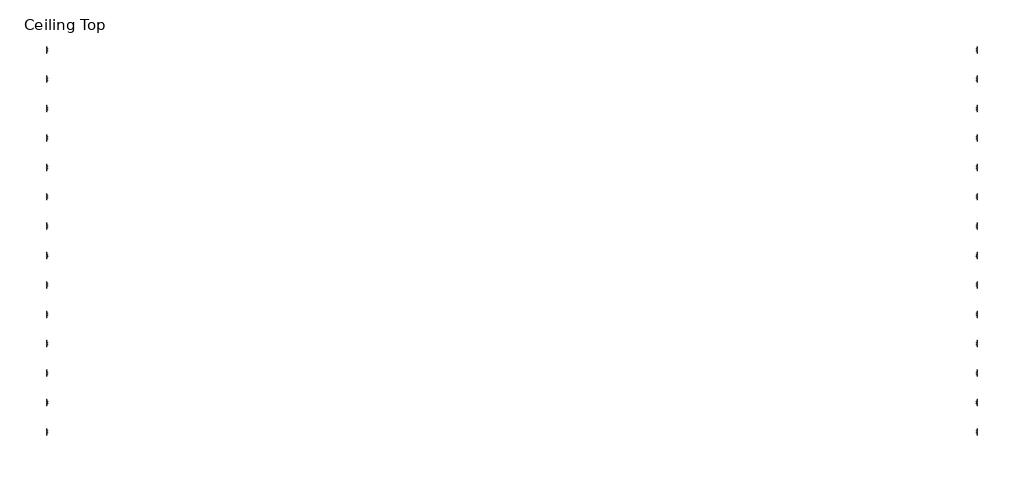
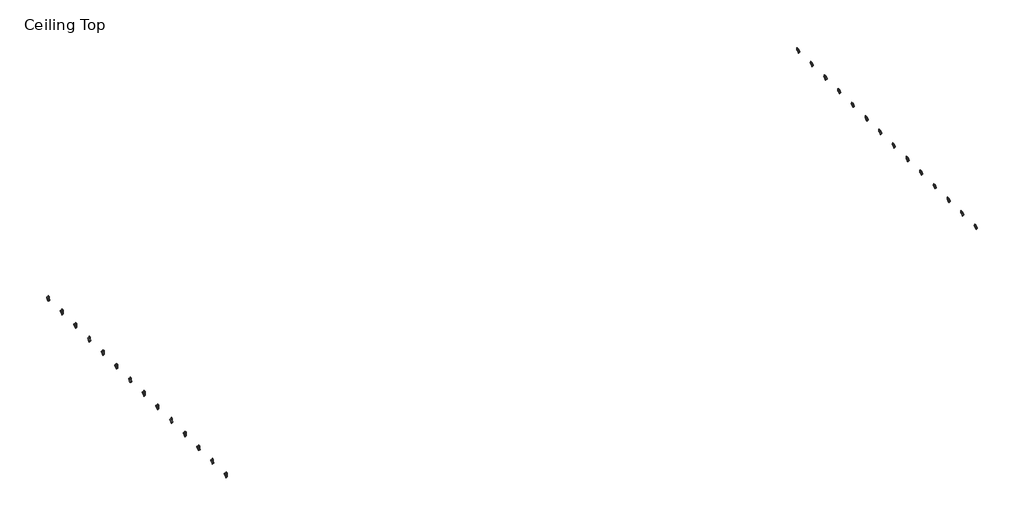
# One storey: 28 proxies.
"""IFC4 building model written with IfcOpenShell, lengths in millimetres."""

import ifcopenshell
import ifcopenshell.guid

model = None  # the IFC model being written
_history = None  # IfcOwnerHistory: only IFC2X3 demands one
_inside = {}  # id of a spatial element -> (the spatial element, [elements in it])
_under = {}  # id of a project, library or spatial element -> (it, [spatial elements below it])
_declared = {}  # id of a project -> (the project, [libraries it declares])
_typed = {}  # id of a type object -> (the type object, [elements of that type])
_made_of = {}  # id of a material, layer set ... -> (it, [elements and type objects made of it])


def new_model(schema):
    """Start an empty IFC model of exactly this schema.

    Asked for "IFC4X3", IfcOpenShell would pick the latest addendum, in which some entities
    have other attributes; the version numbers below select the first issue.
    IFC2X3 requires an IfcOwnerHistory on every rooted entity: one is made here for all.
    """
    global model, _history
    if schema == "IFC4X3":
        model = ifcopenshell.file(schema_version=(4, 3, 0, 0))
    else:
        model = ifcopenshell.file(schema=schema)
    _inside.clear()
    _under.clear()
    _declared.clear()
    _typed.clear()
    _made_of.clear()
    _history = None
    if model.schema == "IFC2X3":
        org = make("IfcOrganization", Name="unknown")
        user = make(
            "IfcPersonAndOrganization",
            ThePerson=make("IfcPerson", FamilyName="unknown"),
            TheOrganization=org,
        )
        app = make(
            "IfcApplication",
            ApplicationDeveloper=org,
            Version="unknown",
            ApplicationFullName="unknown",
            ApplicationIdentifier="unknown",
        )
        _history = make(
            "IfcOwnerHistory",
            OwningUser=user,
            OwningApplication=app,
            ChangeAction="ADDED",
            CreationDate=0,
        )
    return model


def make(cls, **values):
    """One entity of the class cls with the attributes given. An attribute that is None is left unset."""
    return model.create_entity(
        cls, **{name: value for name, value in values.items() if value is not None}
    )


def rooted(cls, **values):
    """An entity with a GlobalId (a new one), such as an element, a storey or a relation."""
    return make(cls, GlobalId=ifcopenshell.guid.new(), OwnerHistory=_history, **values)


def si_unit(unit_type, name, prefix=None):
    """IfcSIUnit, for example si_unit("LENGTHUNIT", "METRE", prefix="MILLI")."""
    return make("IfcSIUnit", UnitType=unit_type, Prefix=prefix, Name=name)


def assignment(units):
    """IfcUnitAssignment: the units of a project."""
    return None if units is None else make("IfcUnitAssignment", Units=units)


def point(xyz):
    """IfcCartesianPoint."""
    return None if xyz is None else make("IfcCartesianPoint", Coordinates=xyz)


def direction(xyz):
    """IfcDirection."""
    return None if xyz is None else make("IfcDirection", DirectionRatios=xyz)


def frame(location, z_axis=None, x_axis=None):
    """IfcAxis2Placement3D, a coordinate frame: its origin and axes. An axis left out is left unset."""
    return make(
        "IfcAxis2Placement3D",
        Location=point(location),
        Axis=direction(z_axis),
        RefDirection=direction(x_axis),
    )


def origin():
    """The frame at (0, 0, 0) with its axes left unset."""
    return frame((0.0, 0.0, 0.0))


def place(relative_to, where):
    """IfcLocalPlacement: puts the frame where relative to a parent placement (None: the world)."""
    return make(
        "IfcLocalPlacement", PlacementRelTo=relative_to, RelativePlacement=where
    )


def context(
    kind, dimensions, precision=None, world=None, true_north=None, identifier=None
):
    """IfcGeometricRepresentationContext, for example the 3D "Model" context."""
    return make(
        "IfcGeometricRepresentationContext",
        ContextIdentifier=identifier,
        ContextType=kind,
        CoordinateSpaceDimension=dimensions,
        Precision=precision,
        WorldCoordinateSystem=world,
        TrueNorth=true_north,
    )


def project(units=None, contexts=None):
    """IfcProject with its units and contexts."""
    return rooted(
        "IfcProject",
        Name="project",
        RepresentationContexts=contexts,
        UnitsInContext=assignment(units),
    )


def spatial(cls, under=None, at=None, **own):
    """A site, building, storey or space (cls), placed at a placement, below another one or the project."""
    s = rooted(cls, ObjectPlacement=at, **own)
    if under is not None:
        _under.setdefault(under.id(), (under, []))[1].append(s)
    return s


def polyline(points):
    """IfcPolyline through the points."""
    return make("IfcPolyline", Points=[point(p) for p in points])


def circle_curve(where, radius):
    """IfcCircle in the frame where."""
    return make("IfcCircle", Position=where, Radius=radius)


def shape(context_of_items, identifier, shape_type, items):
    """IfcShapeRepresentation: the items that make up one representation, for example the "Body"."""
    return make(
        "IfcShapeRepresentation",
        ContextOfItems=context_of_items,
        RepresentationIdentifier=identifier,
        RepresentationType=shape_type,
        Items=items,
    )


def source(mapping_origin, context_of_items, identifier, shape_type, items):
    """IfcRepresentationMap: a shape defined once, which mapped items show again and again."""
    return make(
        "IfcRepresentationMap",
        MappingOrigin=mapping_origin,
        MappedRepresentation=shape(context_of_items, identifier, shape_type, items),
    )


def transform(
    local_origin,
    x_axis=None,
    y_axis=None,
    z_axis=None,
    scale=None,
    scale2=None,
    scale3=None,
    uniform=True,
):
    """IfcCartesianTransformationOperator3D, or its non-uniform kind. x_axis, y_axis, z_axis: its Axis1, 2, 3."""
    if uniform:
        return make(
            "IfcCartesianTransformationOperator3D",
            Axis1=direction(x_axis),
            Axis2=direction(y_axis),
            LocalOrigin=point(local_origin),
            Scale=scale,
            Axis3=direction(z_axis),
        )
    return make(
        "IfcCartesianTransformationOperator3DnonUniform",
        Axis1=direction(x_axis),
        Axis2=direction(y_axis),
        LocalOrigin=point(local_origin),
        Scale=scale,
        Axis3=direction(z_axis),
        Scale2=scale2,
        Scale3=scale3,
    )


def mapped(mapping_source, mapping_target):
    """IfcMappedItem: shows the shape of a source again, moved by a transform."""
    return make(
        "IfcMappedItem", MappingSource=mapping_source, MappingTarget=mapping_target
    )


def made_of(thing, what):
    """Note that an element or type object is made of a material, layer set ...; save() writes the relation."""
    if what is not None:
        _made_of.setdefault(what.id(), (what, []))[1].append(thing)
    return thing


def element(
    cls,
    number,
    at=None,
    inside=None,
    cuts=None,
    type_object=None,
    material=None,
    context=None,
    identifier="Body",
    shape_type=None,
    held_by="IfcProductDefinitionShape",
    body=None,
    shapes=None,
    **own,
):
    """One element of the class cls, such as IfcWall. Its Tag is "e" and its number.

    at: its placement. inside: the storey or other place that contains it. cuts: it is an
    opening in that element (IfcRelVoidsElement). A single representation is given by context,
    identifier, shape_type and body (its items); several are given by shapes. held_by: the class
    of the entity that holds the representations. save() writes the other relations.
    """
    e = rooted(cls, Tag="e%d" % number, ObjectPlacement=at, **own)
    if body is not None:
        shapes = [shape(context, identifier, shape_type, body)]
    if shapes is not None:
        e.Representation = make(held_by, Representations=shapes)
    if inside is not None:
        _inside.setdefault(inside.id(), (inside, []))[1].append(e)
    if cuts is not None:
        rooted(
            "IfcRelVoidsElement", RelatingBuildingElement=cuts, RelatedOpeningElement=e
        )
    if type_object is not None:
        _typed.setdefault(type_object.id(), (type_object, []))[1].append(e)
    return made_of(e, material)


def aggregate(whole, parts):
    """IfcRelAggregates: a whole, such as a stair, and the parts it consists of."""
    return rooted("IfcRelAggregates", RelatingObject=whole, RelatedObjects=parts)


def save(model, path):
    """Write the relations noted so far, then the file.

    IfcRelAggregates (storeys below a building ...), IfcRelContainedInSpatialStructure (elements
    in a storey), IfcRelDefinesByType, IfcRelAssociatesMaterial and IfcRelDeclares: one each for
    every whole, place, type object, material and project.
    """
    for whole, parts in _under.values():
        aggregate(whole, parts)
    for where, things in _inside.values():
        rooted(
            "IfcRelContainedInSpatialStructure",
            RelatedElements=things,
            RelatingStructure=where,
        )
    for kind, things in _typed.values():
        rooted("IfcRelDefinesByType", RelatedObjects=things, RelatingType=kind)
    for what, things in _made_of.values():
        rooted("IfcRelAssociatesMaterial", RelatedObjects=things, RelatingMaterial=what)
    for by, libraries in _declared.values():
        rooted("IfcRelDeclares", RelatingContext=by, RelatedDefinitions=libraries)
    model.write(path)


def plane_surface(at):
    """IfcPlane: the flat surface through the origin of the frame at, square to its z axis."""
    return make("IfcPlane", Position=at)


def revolved_surface(curve, axis_point, axis_direction):
    """IfcSurfaceOfRevolution: the curve turned about the line through axis_point along axis_direction."""
    return make(
        "IfcSurfaceOfRevolution",
        SweptCurve=make("IfcArbitraryOpenProfileDef", ProfileType="CURVE", Curve=curve),
        AxisPosition=make("IfcAxis1Placement", Location=point(axis_point), Axis=direction(axis_direction)),
    )


def advanced_brep(points, edges, surfaces, faces):
    """IfcAdvancedBrep: a solid bounded by faces that lie on surfaces and meet in shared edges.

    An edge is (start, end): straight between two places in points (the first is 0);
    or (start, end, curve); or (start, end, curve, False) where it runs against its curve.
    A face is (place in surfaces, loops), or (place, loops, False) where it looks against
    its surface's normal. A loop lists edges by number (the first is 1), with a minus sign
    where the edge is run from its end to its start. The first loop is the outer one.
    """
    corners = [point(p) for p in points]
    vertices = [make("IfcVertexPoint", VertexGeometry=c) for c in corners]
    made = []
    for start, end, *more in edges:
        made.append(
            make(
                "IfcEdgeCurve",
                EdgeStart=vertices[start],
                EdgeEnd=vertices[end],
                EdgeGeometry=more[0] if more else make("IfcPolyline", Points=[corners[start], corners[end]]),
                SameSense=more[1] if len(more) > 1 else True,
            )
        )
    hull = []
    for where, loops, *sense in faces:
        bounds = []
        for j, loop in enumerate(loops):
            ring = [make("IfcOrientedEdge", EdgeElement=made[abs(k) - 1], Orientation=k > 0) for k in loop]
            bounds.append(
                make(
                    "IfcFaceOuterBound" if j == 0 else "IfcFaceBound",
                    Bound=make("IfcEdgeLoop", EdgeList=ring),
                    Orientation=True,
                )
            )
        hull.append(make("IfcAdvancedFace", Bounds=bounds, FaceSurface=surfaces[where], SameSense=sense[0] if sense else True))
    return make("IfcAdvancedBrep", Outer=make("IfcClosedShell", CfsFaces=hull))


def generic_models_343c88cb(model_context):
    return source(origin(), model_context, "Body", "AdvancedBrep", [
        advanced_brep(
        [(-0.790575, 0.0, 54.76875), (3.171825, 0.0, 54.76875), (3.171825, 1.18872, 54.76875), (-0.790575, 1.18872, 54.76875), (-0.790575, 0.0, 16.66875), (3.171825, 0.0, 16.66875), (3.171825, 1.18872, 16.66875), (-0.790575, 1.18872, 16.66875), (43.659425, 0.0, 10.31875), (47.621825, 0.0, 10.31875), (47.621825, 1.18872, 10.31875), (43.659425, 1.18872, 10.31875), (-45.240575, 0.0, 10.31875), (-41.278175, 0.0, 10.31875), (-41.278175, 1.18872, 10.31875), (-45.240575, 1.18872, 10.31875), (19.84756, 11.902103, -19.05), (19.84756, 15.864503, -19.05), (21.03628, 15.864503, -19.05), (21.03628, 11.902103, -19.05), (19.84756, 11.902103, -36.5125), (19.84756, 15.864503, -36.5125), (21.03628, 15.864503, -36.5125), (21.03628, 11.902103, -36.5125), (19.84756, 11.902103, -53.975), (19.84756, 15.864503, -53.975), (21.03628, 15.864503, -53.975), (21.03628, 11.902103, -53.975), (-21.03628, 11.902103, -57.15), (-21.03628, 15.864503, -57.15), (-19.84756, 15.864503, -57.15), (-19.84756, 11.902103, -57.15), (-21.03628, 11.902103, -39.6875), (-21.03628, 15.864503, -39.6875), (-19.84756, 15.864503, -39.6875), (-19.84756, 11.902103, -39.6875), (-21.03628, 11.902103, -22.225), (-21.03628, 15.864503, -22.225), (-19.84756, 15.864503, -22.225), (-19.84756, 11.902103, -22.225), (23.08225, 0.0, 0.0), (23.08225, 1.18872, 0.0), (23.08225, 1.18872, -3.175), (23.08225, 0.0, -3.175), (21.03628, 0.0, -56.758894), (19.84756, 0.0, -56.758894), (19.84756, 1.698923, -56.758894), (21.03628, 1.698923, -56.758894), (21.03628, 1.18872, -56.758894), (19.84756, 0.0, -3.175), (21.03628, 1.18872, -3.175), (21.03628, 21.820803, -3.175), (19.84756, 21.820803, -3.175), (-23.08225, 1.18872, 0.0), (-23.08225, 1.18872, -3.175), (-21.03628, 1.18872, -3.175), (-21.03628, 1.18872, -56.758894), (-67.071875, 1.18872, -10.723299), (-67.071875, 1.18872, -1.182951), (-4.770174, 1.18872, 61.11875), (4.770174, 1.18872, 61.11875), (67.071875, 1.18872, -1.182951), (67.071875, 1.18872, -10.723299), (19.84756, 21.820803, -73.025), (19.84756, 17.965029, -73.025), (-21.03628, 1.698923, -56.758894), (-19.84756, 1.698923, -56.758894), (-19.84756, 0.0, -56.758894), (-21.03628, 0.0, -56.758894), (67.071875, 0.0, -10.723299), (67.071875, 0.0, -1.182951), (4.770174, 0.0, 61.11875), (-4.770174, 0.0, 61.11875), (-67.071875, 0.0, -1.182951), (-67.071875, 0.0, -10.723299), (-19.84756, 0.0, -3.175), (-23.08225, 0.0, -3.175), (-23.08225, 0.0, 0.0), (-19.84756, 21.820803, -3.175), (-21.03628, 21.820803, -3.175), (21.03628, 17.965029, -73.025), (21.03628, 21.820803, -73.025), (-19.84756, 17.965029, -73.025), (-19.84756, 21.820803, -73.025), (-21.03628, 21.820803, -73.025), (-21.03628, 17.965029, -73.025)],
        [
            (0, 1, circle_curve(frame((1.190625, 0.0, 54.76875), z_axis=(0.0, -1.0, 0.0), x_axis=(-1.0, 0.0, 0.0)), 1.9812)),
            (1, 2),
            (2, 3, circle_curve(frame((1.190625, 1.18872, 54.76875), z_axis=(0.0, 1.0, 0.0), x_axis=(-1.0, 0.0, 0.0)), 1.9812)),
            (3, 0),
            (4, 5, circle_curve(frame((1.190625, 0.0, 16.66875), z_axis=(0.0, -1.0, 0.0), x_axis=(-1.0, 0.0, 0.0)), 1.9812)),
            (5, 6),
            (6, 7, circle_curve(frame((1.190625, 1.18872, 16.66875), z_axis=(0.0, 1.0, 0.0), x_axis=(-1.0, 0.0, 0.0)), 1.9812)),
            (7, 4),
            (8, 9, circle_curve(frame((45.640625, 0.0, 10.31875), z_axis=(0.0, -1.0, 0.0), x_axis=(-1.0, 0.0, 0.0)), 1.9812)),
            (9, 10),
            (10, 11, circle_curve(frame((45.640625, 1.18872, 10.31875), z_axis=(0.0, 1.0, 0.0), x_axis=(-1.0, 0.0, 0.0)), 1.9812)),
            (11, 8),
            (12, 13, circle_curve(frame((-43.259375, 0.0, 10.31875), z_axis=(0.0, -1.0, 0.0), x_axis=(-1.0, 0.0, 0.0)), 1.9812)),
            (13, 14),
            (14, 15, circle_curve(frame((-43.259375, 1.18872, 10.31875), z_axis=(0.0, 1.0, 0.0), x_axis=(-1.0, 0.0, 0.0)), 1.9812)),
            (15, 12),
            (16, 17, circle_curve(frame((19.84756, 13.883303, -19.05), z_axis=(-1.0, 0.0, 0.0), x_axis=(0.0, -1.0, 0.0)), 1.9812)),
            (17, 18),
            (18, 19, circle_curve(frame((21.03628, 13.883303, -19.05), z_axis=(1.0, 0.0, 0.0), x_axis=(0.0, -1.0, 0.0)), 1.9812)),
            (19, 16),
            (20, 21, circle_curve(frame((19.84756, 13.883303, -36.5125), z_axis=(-1.0, 0.0, 0.0), x_axis=(0.0, -1.0, 0.0)), 1.9812)),
            (21, 22),
            (22, 23, circle_curve(frame((21.03628, 13.883303, -36.5125), z_axis=(1.0, 0.0, 0.0), x_axis=(0.0, -1.0, 0.0)), 1.9812)),
            (23, 20),
            (24, 25, circle_curve(frame((19.84756, 13.883303, -53.975), z_axis=(-1.0, 0.0, 0.0), x_axis=(0.0, -1.0, 0.0)), 1.9812)),
            (25, 26),
            (26, 27, circle_curve(frame((21.03628, 13.883303, -53.975), z_axis=(1.0, 0.0, 0.0), x_axis=(0.0, -1.0, 0.0)), 1.9812)),
            (27, 24),
            (28, 29, circle_curve(frame((-21.03628, 13.883303, -57.15), z_axis=(-1.0, 0.0, 0.0), x_axis=(0.0, -1.0, 0.0)), 1.9812)),
            (29, 30),
            (30, 31, circle_curve(frame((-19.84756, 13.883303, -57.15), z_axis=(1.0, 0.0, 0.0), x_axis=(0.0, -1.0, 0.0)), 1.9812)),
            (31, 28),
            (32, 33, circle_curve(frame((-21.03628, 13.883303, -39.6875), z_axis=(-1.0, 0.0, 0.0), x_axis=(0.0, -1.0, 0.0)), 1.9812)),
            (33, 34),
            (34, 35, circle_curve(frame((-19.84756, 13.883303, -39.6875), z_axis=(1.0, 0.0, 0.0), x_axis=(0.0, -1.0, 0.0)), 1.9812)),
            (35, 32),
            (36, 37, circle_curve(frame((-21.03628, 13.883303, -22.225), z_axis=(-1.0, 0.0, 0.0), x_axis=(0.0, -1.0, 0.0)), 1.9812)),
            (37, 38),
            (38, 39, circle_curve(frame((-19.84756, 13.883303, -22.225), z_axis=(1.0, 0.0, 0.0), x_axis=(0.0, -1.0, 0.0)), 1.9812)),
            (39, 36),
            (40, 41),
            (41, 42),
            (42, 43),
            (43, 40),
            (44, 45),
            (45, 46),
            (46, 47),
            (47, 48),
            (48, 44),
            (49, 43),
            (42, 50),
            (50, 51),
            (51, 52),
            (52, 49),
            (53, 54),
            (54, 55),
            (55, 56),
            (56, 57),
            (57, 58),
            (58, 59),
            (59, 60),
            (60, 61),
            (61, 62),
            (62, 48),
            (48, 50),
            (41, 53),
            (14, 15, circle_curve(frame((-43.259375, 1.18872, 10.31875), z_axis=(0.0, -1.0, 0.0), x_axis=(-1.0, 0.0, 0.0)), 1.9812)),
            (10, 11, circle_curve(frame((45.640625, 1.18872, 10.31875), z_axis=(0.0, -1.0, 0.0), x_axis=(-1.0, 0.0, 0.0)), 1.9812)),
            (6, 7, circle_curve(frame((1.190625, 1.18872, 16.66875), z_axis=(0.0, -1.0, 0.0), x_axis=(-1.0, 0.0, 0.0)), 1.9812)),
            (2, 3, circle_curve(frame((1.190625, 1.18872, 54.76875), z_axis=(0.0, -1.0, 0.0), x_axis=(-1.0, 0.0, 0.0)), 1.9812)),
            (45, 49),
            (52, 63),
            (63, 64),
            (64, 46),
            (16, 17, circle_curve(frame((19.84756, 13.883303, -19.05), z_axis=(1.0, 0.0, 0.0), x_axis=(0.0, -1.0, 0.0)), 1.9812)),
            (20, 21, circle_curve(frame((19.84756, 13.883303, -36.5125), z_axis=(1.0, 0.0, 0.0), x_axis=(0.0, -1.0, 0.0)), 1.9812)),
            (24, 25, circle_curve(frame((19.84756, 13.883303, -53.975), z_axis=(1.0, 0.0, 0.0), x_axis=(0.0, -1.0, 0.0)), 1.9812)),
            (56, 65),
            (65, 66),
            (66, 67),
            (67, 68),
            (68, 56),
            (44, 69),
            (69, 70),
            (70, 71),
            (71, 72),
            (72, 73),
            (73, 74),
            (74, 68),
            (67, 75),
            (75, 76),
            (76, 77),
            (77, 40),
            (0, 1, circle_curve(frame((1.190625, 0.0, 54.76875), z_axis=(0.0, 1.0, 0.0), x_axis=(-1.0, 0.0, 0.0)), 1.9812)),
            (4, 5, circle_curve(frame((1.190625, 0.0, 16.66875), z_axis=(0.0, 1.0, 0.0), x_axis=(-1.0, 0.0, 0.0)), 1.9812)),
            (8, 9, circle_curve(frame((45.640625, 0.0, 10.31875), z_axis=(0.0, 1.0, 0.0), x_axis=(-1.0, 0.0, 0.0)), 1.9812)),
            (12, 13, circle_curve(frame((-43.259375, 0.0, 10.31875), z_axis=(0.0, 1.0, 0.0), x_axis=(-1.0, 0.0, 0.0)), 1.9812)),
            (74, 57),
            (76, 54),
            (53, 77),
            (75, 78),
            (78, 79),
            (79, 55),
            (64, 80),
            (80, 47),
            (80, 81),
            (81, 51),
            (26, 27, circle_curve(frame((21.03628, 13.883303, -53.975), z_axis=(-1.0, 0.0, 0.0), x_axis=(0.0, -1.0, 0.0)), 1.9812)),
            (22, 23, circle_curve(frame((21.03628, 13.883303, -36.5125), z_axis=(-1.0, 0.0, 0.0), x_axis=(0.0, -1.0, 0.0)), 1.9812)),
            (18, 19, circle_curve(frame((21.03628, 13.883303, -19.05), z_axis=(-1.0, 0.0, 0.0), x_axis=(0.0, -1.0, 0.0)), 1.9812)),
            (66, 82),
            (82, 83),
            (83, 78),
            (38, 39, circle_curve(frame((-19.84756, 13.883303, -22.225), z_axis=(-1.0, 0.0, 0.0), x_axis=(0.0, -1.0, 0.0)), 1.9812)),
            (34, 35, circle_curve(frame((-19.84756, 13.883303, -39.6875), z_axis=(-1.0, 0.0, 0.0), x_axis=(0.0, -1.0, 0.0)), 1.9812)),
            (30, 31, circle_curve(frame((-19.84756, 13.883303, -57.15), z_axis=(-1.0, 0.0, 0.0), x_axis=(0.0, -1.0, 0.0)), 1.9812)),
            (79, 84),
            (84, 85),
            (85, 65),
            (28, 29, circle_curve(frame((-21.03628, 13.883303, -57.15), z_axis=(1.0, 0.0, 0.0), x_axis=(0.0, -1.0, 0.0)), 1.9812)),
            (32, 33, circle_curve(frame((-21.03628, 13.883303, -39.6875), z_axis=(1.0, 0.0, 0.0), x_axis=(0.0, -1.0, 0.0)), 1.9812)),
            (36, 37, circle_curve(frame((-21.03628, 13.883303, -22.225), z_axis=(1.0, 0.0, 0.0), x_axis=(0.0, -1.0, 0.0)), 1.9812)),
            (85, 82),
            (72, 59),
            (58, 73),
            (84, 83),
            (81, 63),
            (62, 69),
            (61, 70),
            (60, 71),
        ],
        [
            revolved_surface(polyline([(-0.790575, 0.0, 54.76875), (-0.790575, 1.18872, 54.76875)]), (1.190625, 1.18872, 54.76875), (0.0, -1.0, 0.0)),
            revolved_surface(polyline([(-0.790575, 0.0, 16.66875), (-0.790575, 1.18872, 16.66875)]), (1.190625, 1.18872, 16.66875), (0.0, -1.0, 0.0)),
            revolved_surface(polyline([(43.659425, 0.0, 10.31875), (43.659425, 1.18872, 10.31875)]), (45.640625, 1.18872, 10.31875), (0.0, -1.0, 0.0)),
            revolved_surface(polyline([(-45.240575, 0.0, 10.31875), (-45.240575, 1.18872, 10.31875)]), (-43.259375, 1.18872, 10.31875), (0.0, -1.0, 0.0)),
            revolved_surface(polyline([(19.84756, 11.902103, -19.05), (21.03628, 11.902103, -19.05)]), (21.03628, 13.883303, -19.05), (-1.0, 0.0, 0.0)),
            revolved_surface(polyline([(19.84756, 11.902103, -36.5125), (21.03628, 11.902103, -36.5125)]), (21.03628, 13.883303, -36.5125), (-1.0, 0.0, 0.0)),
            revolved_surface(polyline([(19.84756, 11.902103, -53.975), (21.03628, 11.902103, -53.975)]), (21.03628, 13.883303, -53.975), (-1.0, 0.0, 0.0)),
            revolved_surface(polyline([(-21.03628, 11.902103, -57.15), (-19.84756, 11.902103, -57.15)]), (-19.84756, 13.883303, -57.15), (-1.0, 0.0, 0.0)),
            revolved_surface(polyline([(-21.03628, 11.902103, -39.6875), (-19.84756, 11.902103, -39.6875)]), (-19.84756, 13.883303, -39.6875), (-1.0, 0.0, 0.0)),
            revolved_surface(polyline([(-21.03628, 11.902103, -22.225), (-19.84756, 11.902103, -22.225)]), (-19.84756, 13.883303, -22.225), (-1.0, 0.0, 0.0)),
            plane_surface(frame((23.08225, 1.18872, -3.175), z_axis=(-1.0, 0.0, 0.0), x_axis=(0.0, 0.0, 1.0))),
            plane_surface(frame((19.84756, 0.0, -56.758894), z_axis=(0.0, 0.0, -1.0), x_axis=(1.0, 0.0, 0.0))),
            plane_surface(frame((21.03628, 1.240453, -3.175), z_axis=(0.0, 0.0, 1.0), x_axis=(1.0, 0.0, 0.0))),
            plane_surface(frame((0.0, 1.18872, -12.3047323), z_axis=(0.0, 1.0, 0.0), x_axis=(1.0, 0.0, 0.0))),
            plane_surface(frame((19.84756, 22.735203, -12.3047323), z_axis=(-1.0, 0.0, 0.0), x_axis=(0.0, -1.0, 0.0))),
            plane_surface(frame((-19.84756, 0.0, -56.758894), z_axis=(0.0, 0.0, -1.0), x_axis=(-1.0, 0.0, 0.0))),
            plane_surface(frame((0.0, 0.0, -12.3047323), z_axis=(0.0, -1.0, 0.0), x_axis=(1.0, 0.0, 0.0))),
            plane_surface(frame((-67.071875, 1.18872, -10.723299), z_axis=(-0.7071067811865432, 0.0, -0.7071067811865518), x_axis=(0.0, -1.0, 0.0))),
            plane_surface(frame((-23.08225, 1.18872, -3.175), z_axis=(1.0, 0.0, 0.0), x_axis=(0.0, 0.0, 1.0))),
            plane_surface(frame((-21.03628, 21.820803, -3.175), z_axis=(0.0, 0.0, 1.0), x_axis=(-1.0, 0.0, 0.0))),
            plane_surface(frame((21.03628, 17.965029, -73.025), z_axis=(0.0, -0.7071067811865476, -0.7071067811865475), x_axis=(1.0, 0.0, 0.0))),
            plane_surface(frame((21.03628, 22.735203, -12.3047323), z_axis=(1.0, 0.0, 0.0), x_axis=(0.0, -1.0, 0.0))),
            plane_surface(frame((-19.84756, 22.735203, -12.3047323), z_axis=(1.0, 0.0, 0.0), x_axis=(0.0, 1.0, 0.0))),
            plane_surface(frame((-21.03628, 22.735203, -12.3047323), z_axis=(-1.0, 0.0, 0.0), x_axis=(0.0, 1.0, 0.0))),
            plane_surface(frame((-4.770174, 1.18872, 61.11875), z_axis=(-0.7071067811865518, 0.0, 0.7071067811865434), x_axis=(0.0, -1.0, 0.0))),
            plane_surface(frame((-67.071875, 1.18872, -1.182951), z_axis=(-1.0, 0.0, 0.0), x_axis=(0.0, -1.0, 0.0))),
            plane_surface(frame((-21.03628, 17.965029, -73.025), z_axis=(0.0, 0.0, -1.0), x_axis=(1.0, 0.0, 0.0))),
            plane_surface(frame((-21.03628, 21.820803, -73.025), z_axis=(0.0, 1.0, 0.0), x_axis=(-1.0, 0.0, 0.0))),
            plane_surface(frame((-21.49475, 1.18872, 0.0), z_axis=(0.0, 0.0, -1.0), x_axis=(0.0, -1.0, 0.0))),
            plane_surface(frame((21.03628, 21.820803, -3.175), z_axis=(0.0, 1.0, 0.0), x_axis=(-1.0, 0.0, 0.0))),
            plane_surface(frame((21.03628, 21.820803, -73.025), z_axis=(0.0, 0.0, -1.0), x_axis=(-1.0, 0.0, 0.0))),
            plane_surface(frame((4.770174, 1.18872, -73.025), z_axis=(0.7071067811865519, 0.0, -0.7071067811865431), x_axis=(0.0, 1.0, 0.0))),
            plane_surface(frame((67.071875, 1.18872, -10.723299), z_axis=(1.0, 0.0, 0.0), x_axis=(0.0, 1.0, 0.0))),
            plane_surface(frame((67.071875, 1.18872, -1.182951), z_axis=(0.707106781186543, 0.0, 0.707106781186552), x_axis=(0.0, 1.0, 0.0))),
            plane_surface(frame((4.770174, 1.18872, 61.11875), z_axis=(0.0, 0.0, 1.0), x_axis=(0.0, 1.0, 0.0))),
        ],
        [
            (0, [[1, 2, 3, 4]]),
            (1, [[5, 6, 7, 8]]),
            (2, [[9, 10, 11, 12]]),
            (3, [[13, 14, 15, 16]]),
            (4, [[17, 18, 19, 20]]),
            (5, [[21, 22, 23, 24]]),
            (6, [[25, 26, 27, 28]]),
            (7, [[29, 30, 31, 32]]),
            (8, [[33, 34, 35, 36]]),
            (9, [[37, 38, 39, 40]]),
            (10, [[41, 42, 43, 44]]),
            (11, [[45, 46, 47, 48, 49]]),
            (12, [[50, -43, 51, 52, 53, 54]]),
            (13, [[55, 56, 57, 58, 59, 60, 61, 62, 63, 64, 65, -51, -42, 66], [67, -15], [68, -11], [69, -7], [70, -3]]),
            (14, [[71, -54, 72, 73, 74, -46], [-17, 75], [-21, 76], [-25, 77]]),
            (15, [[78, 79, 80, 81, 82]]),
            (16, [[-44, -50, -71, -45, 83, 84, 85, 86, 87, 88, 89, -81, 90, 91, 92, 93], [-1, 94], [-5, 95], [-9, 96], [-13, 97]]),
            (17, [[-89, 98, -58, -82]]),
            (18, [[99, -55, 100, -92]]),
            (19, [[-56, -99, -91, 101, 102, 103]]),
            (20, [[-47, -74, 104, 105]]),
            (21, [[-48, -105, 106, 107, -52, -65], [108, -27], [109, -23], [110, -19]]),
            (22, [[111, 112, 113, -101, -90, -80], [114, -39], [115, -35], [116, -31]]),
            (23, [[-57, -103, 117, 118, 119, -78], [-29, 120], [-33, 121], [-37, 122]]),
            (9, [[-114, -38, -122, -40]]),
            (8, [[-115, -34, -121, -36]]),
            (7, [[-116, -30, -120, -32]]),
            (6, [[-108, -26, -77, -28]]),
            (5, [[-109, -22, -76, -24]]),
            (4, [[-110, -18, -75, -20]]),
            (20, [[-79, -119, 123, -111]]),
            (3, [[-67, -14, -97, -16]]),
            (2, [[-68, -10, -96, -12]]),
            (1, [[-69, -6, -95, -8]]),
            (0, [[-70, -2, -94, -4]]),
            (24, [[124, -60, 125, -87]]),
            (25, [[-125, -59, -98, -88]]),
            (26, [[-123, -118, 126, -112]]),
            (27, [[-126, -117, -102, -113]]),
            (28, [[-41, -93, -100, -66]]),
            (29, [[-53, -107, 127, -72]]),
            (30, [[-127, -106, -104, -73]]),
            (31, [[-64, 128, -83, -49]]),
            (32, [[-128, -63, 129, -84]]),
            (33, [[-129, -62, 130, -85]]),
            (34, [[-130, -61, -124, -86]]),
        ],
    ),
    ])


def generic_models_ac6e08b7(model_context):
    return source(origin(), model_context, "Body", "AdvancedBrep", [
        advanced_brep(
        [(-0.790575, 0.0, 54.76875), (-0.790575, -1.18872, 54.76875), (3.171825, -1.18872, 54.76875), (3.171825, 0.0, 54.76875), (-0.790575, 0.0, 16.66875), (-0.790575, -1.18872, 16.66875), (3.171825, -1.18872, 16.66875), (3.171825, 0.0, 16.66875), (43.659425, 0.0, 10.31875), (43.659425, -1.18872, 10.31875), (47.621825, -1.18872, 10.31875), (47.621825, 0.0, 10.31875), (-45.240575, 0.0, 10.31875), (-45.240575, -1.18872, 10.31875), (-41.278175, -1.18872, 10.31875), (-41.278175, 0.0, 10.31875), (19.84756, -11.902103, -19.05), (21.03628, -11.902103, -19.05), (21.03628, -15.864503, -19.05), (19.84756, -15.864503, -19.05), (19.84756, -11.902103, -36.5125), (21.03628, -11.902103, -36.5125), (21.03628, -15.864503, -36.5125), (19.84756, -15.864503, -36.5125), (19.84756, -11.902103, -53.975), (21.03628, -11.902103, -53.975), (21.03628, -15.864503, -53.975), (19.84756, -15.864503, -53.975), (-21.03628, -11.902103, -57.15), (-19.84756, -11.902103, -57.15), (-19.84756, -15.864503, -57.15), (-21.03628, -15.864503, -57.15), (-21.03628, -11.902103, -39.6875), (-19.84756, -11.902103, -39.6875), (-19.84756, -15.864503, -39.6875), (-21.03628, -15.864503, -39.6875), (-21.03628, -11.902103, -22.225), (-19.84756, -11.902103, -22.225), (-19.84756, -15.864503, -22.225), (-21.03628, -15.864503, -22.225), (23.08225, 0.0, 0.0), (23.08225, 0.0, -3.175), (23.08225, -1.18872, -3.175), (23.08225, -1.18872, 0.0), (21.03628, 0.0, -56.758894), (21.03628, -1.18872, -56.758894), (21.03628, -1.698923, -56.758894), (19.84756, -1.698923, -56.758894), (19.84756, 0.0, -56.758894), (19.84756, 0.0, -3.175), (19.84756, -21.820803, -3.175), (21.03628, -21.820803, -3.175), (21.03628, -1.18872, -3.175), (-23.08225, -1.18872, 0.0), (67.071875, -1.18872, -10.723299), (67.071875, -1.18872, -1.182951), (4.770174, -1.18872, 61.11875), (-4.770174, -1.18872, 61.11875), (-67.071875, -1.18872, -1.182951), (-67.071875, -1.18872, -10.723299), (-21.03628, -1.18872, -56.758894), (-21.03628, -1.18872, -3.175), (-23.08225, -1.18872, -3.175), (19.84756, -17.965029, -73.025), (19.84756, -21.820803, -73.025), (-21.03628, 0.0, -56.758894), (-19.84756, 0.0, -56.758894), (-19.84756, -1.698923, -56.758894), (-21.03628, -1.698923, -56.758894), (-23.08225, 0.0, 0.0), (-23.08225, 0.0, -3.175), (-19.84756, 0.0, -3.175), (-67.071875, 0.0, -10.723299), (-67.071875, 0.0, -1.182951), (-4.770174, 0.0, 61.11875), (4.770174, 0.0, 61.11875), (67.071875, 0.0, -1.182951), (67.071875, 0.0, -10.723299), (-21.03628, -21.820803, -3.175), (-19.84756, -21.820803, -3.175), (21.03628, -17.965029, -73.025), (21.03628, -21.820803, -73.025), (-19.84756, -21.820803, -73.025), (-19.84756, -17.965029, -73.025), (-21.03628, -17.965029, -73.025), (-21.03628, -21.820803, -73.025)],
        [
            (0, 1),
            (1, 2, circle_curve(frame((1.190625, -1.18872, 54.76875), z_axis=(0.0, -1.0, 0.0), x_axis=(-1.0, 0.0, 0.0)), 1.9812)),
            (2, 3),
            (3, 0, circle_curve(frame((1.190625, 0.0, 54.76875), z_axis=(0.0, 1.0, 0.0), x_axis=(-1.0, 0.0, 0.0)), 1.9812)),
            (4, 5),
            (5, 6, circle_curve(frame((1.190625, -1.18872, 16.66875), z_axis=(0.0, -1.0, 0.0), x_axis=(-1.0, 0.0, 0.0)), 1.9812)),
            (6, 7),
            (7, 4, circle_curve(frame((1.190625, 0.0, 16.66875), z_axis=(0.0, 1.0, 0.0), x_axis=(-1.0, 0.0, 0.0)), 1.9812)),
            (8, 9),
            (9, 10, circle_curve(frame((45.640625, -1.18872, 10.31875), z_axis=(0.0, -1.0, 0.0), x_axis=(-1.0, 0.0, 0.0)), 1.9812)),
            (10, 11),
            (11, 8, circle_curve(frame((45.640625, 0.0, 10.31875), z_axis=(0.0, 1.0, 0.0), x_axis=(-1.0, 0.0, 0.0)), 1.9812)),
            (12, 13),
            (13, 14, circle_curve(frame((-43.259375, -1.18872, 10.31875), z_axis=(0.0, -1.0, 0.0), x_axis=(-1.0, 0.0, 0.0)), 1.9812)),
            (14, 15),
            (15, 12, circle_curve(frame((-43.259375, 0.0, 10.31875), z_axis=(0.0, 1.0, 0.0), x_axis=(-1.0, 0.0, 0.0)), 1.9812)),
            (16, 17),
            (17, 18, circle_curve(frame((21.03628, -13.883303, -19.05), z_axis=(1.0, 0.0, 0.0), x_axis=(0.0, 1.0, 0.0)), 1.9812)),
            (18, 19),
            (19, 16, circle_curve(frame((19.84756, -13.883303, -19.05), z_axis=(-1.0, 0.0, 0.0), x_axis=(0.0, 1.0, 0.0)), 1.9812)),
            (20, 21),
            (21, 22, circle_curve(frame((21.03628, -13.883303, -36.5125), z_axis=(1.0, 0.0, 0.0), x_axis=(0.0, 1.0, 0.0)), 1.9812)),
            (22, 23),
            (23, 20, circle_curve(frame((19.84756, -13.883303, -36.5125), z_axis=(-1.0, 0.0, 0.0), x_axis=(0.0, 1.0, 0.0)), 1.9812)),
            (24, 25),
            (25, 26, circle_curve(frame((21.03628, -13.883303, -53.975), z_axis=(1.0, 0.0, 0.0), x_axis=(0.0, 1.0, 0.0)), 1.9812)),
            (26, 27),
            (27, 24, circle_curve(frame((19.84756, -13.883303, -53.975), z_axis=(-1.0, 0.0, 0.0), x_axis=(0.0, 1.0, 0.0)), 1.9812)),
            (28, 29),
            (29, 30, circle_curve(frame((-19.84756, -13.883303, -57.15), z_axis=(1.0, 0.0, 0.0), x_axis=(0.0, 1.0, 0.0)), 1.9812)),
            (30, 31),
            (31, 28, circle_curve(frame((-21.03628, -13.883303, -57.15), z_axis=(-1.0, 0.0, 0.0), x_axis=(0.0, 1.0, 0.0)), 1.9812)),
            (32, 33),
            (33, 34, circle_curve(frame((-19.84756, -13.883303, -39.6875), z_axis=(1.0, 0.0, 0.0), x_axis=(0.0, 1.0, 0.0)), 1.9812)),
            (34, 35),
            (35, 32, circle_curve(frame((-21.03628, -13.883303, -39.6875), z_axis=(-1.0, 0.0, 0.0), x_axis=(0.0, 1.0, 0.0)), 1.9812)),
            (36, 37),
            (37, 38, circle_curve(frame((-19.84756, -13.883303, -22.225), z_axis=(1.0, 0.0, 0.0), x_axis=(0.0, 1.0, 0.0)), 1.9812)),
            (38, 39),
            (39, 36, circle_curve(frame((-21.03628, -13.883303, -22.225), z_axis=(-1.0, 0.0, 0.0), x_axis=(0.0, 1.0, 0.0)), 1.9812)),
            (40, 41),
            (41, 42),
            (42, 43),
            (43, 40),
            (44, 45),
            (45, 46),
            (46, 47),
            (47, 48),
            (48, 44),
            (49, 50),
            (50, 51),
            (51, 52),
            (52, 42),
            (41, 49),
            (53, 43),
            (52, 45),
            (45, 54),
            (54, 55),
            (55, 56),
            (56, 57),
            (57, 58),
            (58, 59),
            (59, 60),
            (60, 61),
            (61, 62),
            (62, 53),
            (1, 2, circle_curve(frame((1.190625, -1.18872, 54.76875), z_axis=(0.0, 1.0, 0.0), x_axis=(-1.0, 0.0, 0.0)), 1.9812)),
            (5, 6, circle_curve(frame((1.190625, -1.18872, 16.66875), z_axis=(0.0, 1.0, 0.0), x_axis=(-1.0, 0.0, 0.0)), 1.9812)),
            (9, 10, circle_curve(frame((45.640625, -1.18872, 10.31875), z_axis=(0.0, 1.0, 0.0), x_axis=(-1.0, 0.0, 0.0)), 1.9812)),
            (13, 14, circle_curve(frame((-43.259375, -1.18872, 10.31875), z_axis=(0.0, 1.0, 0.0), x_axis=(-1.0, 0.0, 0.0)), 1.9812)),
            (47, 63),
            (63, 64),
            (64, 50),
            (49, 48),
            (19, 16, circle_curve(frame((19.84756, -13.883303, -19.05), z_axis=(1.0, 0.0, 0.0), x_axis=(0.0, 1.0, 0.0)), 1.9812)),
            (23, 20, circle_curve(frame((19.84756, -13.883303, -36.5125), z_axis=(1.0, 0.0, 0.0), x_axis=(0.0, 1.0, 0.0)), 1.9812)),
            (27, 24, circle_curve(frame((19.84756, -13.883303, -53.975), z_axis=(1.0, 0.0, 0.0), x_axis=(0.0, 1.0, 0.0)), 1.9812)),
            (60, 65),
            (65, 66),
            (66, 67),
            (67, 68),
            (68, 60),
            (40, 69),
            (69, 70),
            (70, 71),
            (71, 66),
            (65, 72),
            (72, 73),
            (73, 74),
            (74, 75),
            (75, 76),
            (76, 77),
            (77, 44),
            (3, 0, circle_curve(frame((1.190625, 0.0, 54.76875), z_axis=(0.0, -1.0, 0.0), x_axis=(-1.0, 0.0, 0.0)), 1.9812)),
            (7, 4, circle_curve(frame((1.190625, 0.0, 16.66875), z_axis=(0.0, -1.0, 0.0), x_axis=(-1.0, 0.0, 0.0)), 1.9812)),
            (11, 8, circle_curve(frame((45.640625, 0.0, 10.31875), z_axis=(0.0, -1.0, 0.0), x_axis=(-1.0, 0.0, 0.0)), 1.9812)),
            (15, 12, circle_curve(frame((-43.259375, 0.0, 10.31875), z_axis=(0.0, -1.0, 0.0), x_axis=(-1.0, 0.0, 0.0)), 1.9812)),
            (59, 72),
            (69, 53),
            (62, 70),
            (61, 78),
            (78, 79),
            (79, 71),
            (46, 80),
            (80, 63),
            (51, 81),
            (81, 80),
            (17, 18, circle_curve(frame((21.03628, -13.883303, -19.05), z_axis=(-1.0, 0.0, 0.0), x_axis=(0.0, 1.0, 0.0)), 1.9812)),
            (21, 22, circle_curve(frame((21.03628, -13.883303, -36.5125), z_axis=(-1.0, 0.0, 0.0), x_axis=(0.0, 1.0, 0.0)), 1.9812)),
            (25, 26, circle_curve(frame((21.03628, -13.883303, -53.975), z_axis=(-1.0, 0.0, 0.0), x_axis=(0.0, 1.0, 0.0)), 1.9812)),
            (79, 82),
            (82, 83),
            (83, 67),
            (29, 30, circle_curve(frame((-19.84756, -13.883303, -57.15), z_axis=(-1.0, 0.0, 0.0), x_axis=(0.0, 1.0, 0.0)), 1.9812)),
            (33, 34, circle_curve(frame((-19.84756, -13.883303, -39.6875), z_axis=(-1.0, 0.0, 0.0), x_axis=(0.0, 1.0, 0.0)), 1.9812)),
            (37, 38, circle_curve(frame((-19.84756, -13.883303, -22.225), z_axis=(-1.0, 0.0, 0.0), x_axis=(0.0, 1.0, 0.0)), 1.9812)),
            (68, 84),
            (84, 85),
            (85, 78),
            (31, 28, circle_curve(frame((-21.03628, -13.883303, -57.15), z_axis=(1.0, 0.0, 0.0), x_axis=(0.0, 1.0, 0.0)), 1.9812)),
            (35, 32, circle_curve(frame((-21.03628, -13.883303, -39.6875), z_axis=(1.0, 0.0, 0.0), x_axis=(0.0, 1.0, 0.0)), 1.9812)),
            (39, 36, circle_curve(frame((-21.03628, -13.883303, -22.225), z_axis=(1.0, 0.0, 0.0), x_axis=(0.0, 1.0, 0.0)), 1.9812)),
            (83, 84),
            (73, 58),
            (57, 74),
            (82, 85),
            (64, 81),
            (77, 54),
            (76, 55),
            (75, 56),
        ],
        [
            revolved_surface(polyline([(-0.790575, 0.0, 54.76875), (-0.790575, -1.18872, 54.76875)]), (1.190625, -1.18872, 54.76875), (0.0, 1.0, 0.0)),
            revolved_surface(polyline([(-0.790575, 0.0, 16.66875), (-0.790575, -1.18872, 16.66875)]), (1.190625, -1.18872, 16.66875), (0.0, 1.0, 0.0)),
            revolved_surface(polyline([(43.659425, 0.0, 10.31875), (43.659425, -1.18872, 10.31875)]), (45.640625, -1.18872, 10.31875), (0.0, 1.0, 0.0)),
            revolved_surface(polyline([(-45.240575, 0.0, 10.31875), (-45.240575, -1.18872, 10.31875)]), (-43.259375, -1.18872, 10.31875), (0.0, 1.0, 0.0)),
            revolved_surface(polyline([(19.84756, -11.902103, -19.05), (21.03628, -11.902103, -19.05)]), (21.03628, -13.883303, -19.05), (-1.0, 0.0, 0.0)),
            revolved_surface(polyline([(19.84756, -11.902103, -36.5125), (21.03628, -11.902103, -36.5125)]), (21.03628, -13.883303, -36.5125), (-1.0, 0.0, 0.0)),
            revolved_surface(polyline([(19.84756, -11.902103, -53.975), (21.03628, -11.902103, -53.975)]), (21.03628, -13.883303, -53.975), (-1.0, 0.0, 0.0)),
            revolved_surface(polyline([(-21.03628, -11.902103, -57.15), (-19.84756, -11.902103, -57.15)]), (-19.84756, -13.883303, -57.15), (-1.0, 0.0, 0.0)),
            revolved_surface(polyline([(-21.03628, -11.902103, -39.6875), (-19.84756, -11.902103, -39.6875)]), (-19.84756, -13.883303, -39.6875), (-1.0, 0.0, 0.0)),
            revolved_surface(polyline([(-21.03628, -11.902103, -22.225), (-19.84756, -11.902103, -22.225)]), (-19.84756, -13.883303, -22.225), (-1.0, 0.0, 0.0)),
            plane_surface(frame((23.08225, -1.18872, -3.175), z_axis=(-1.0, 0.0, 0.0), x_axis=(0.0, 0.0, 1.0))),
            plane_surface(frame((19.84756, 0.0, -56.758894), z_axis=(0.0, 0.0, -1.0), x_axis=(1.0, 0.0, 0.0))),
            plane_surface(frame((21.03628, -1.240453, -3.175), z_axis=(0.0, 0.0, 1.0), x_axis=(1.0, 0.0, 0.0))),
            plane_surface(frame((0.0, -1.18872, -12.3047323), z_axis=(0.0, -1.0, 0.0), x_axis=(1.0, 0.0, 0.0))),
            plane_surface(frame((19.84756, -22.735203, -12.3047323), z_axis=(-1.0, 0.0, 0.0), x_axis=(0.0, 1.0, 0.0))),
            plane_surface(frame((-19.84756, 0.0, -56.758894), z_axis=(0.0, 0.0, -1.0), x_axis=(-1.0, 0.0, 0.0))),
            plane_surface(frame((0.0, 0.0, -12.3047323), z_axis=(0.0, 1.0, 0.0), x_axis=(1.0, 0.0, 0.0))),
            plane_surface(frame((-67.071875, -1.18872, -10.723299), z_axis=(-0.7071067811865432, 0.0, -0.7071067811865518), x_axis=(0.0, 1.0, 0.0))),
            plane_surface(frame((-23.08225, -1.18872, -3.175), z_axis=(1.0, 0.0, 0.0), x_axis=(0.0, 0.0, 1.0))),
            plane_surface(frame((-21.03628, -21.820803, -3.175), z_axis=(0.0, 0.0, 1.0), x_axis=(-1.0, 0.0, 0.0))),
            plane_surface(frame((21.03628, -17.965029, -73.025), z_axis=(0.0, 0.7071067811865476, -0.7071067811865475), x_axis=(1.0, 0.0, 0.0))),
            plane_surface(frame((21.03628, -22.735203, -12.3047323), z_axis=(1.0, 0.0, 0.0), x_axis=(0.0, 1.0, 0.0))),
            plane_surface(frame((-19.84756, -22.735203, -12.3047323), z_axis=(1.0, 0.0, 0.0), x_axis=(0.0, -1.0, 0.0))),
            plane_surface(frame((-21.03628, -22.735203, -12.3047323), z_axis=(-1.0, 0.0, 0.0), x_axis=(0.0, -1.0, 0.0))),
            plane_surface(frame((-4.770174, -1.18872, 61.11875), z_axis=(-0.7071067811865518, 0.0, 0.7071067811865434), x_axis=(0.0, 1.0, 0.0))),
            plane_surface(frame((-67.071875, -1.18872, -1.182951), z_axis=(-1.0, 0.0, 0.0), x_axis=(0.0, 1.0, 0.0))),
            plane_surface(frame((-21.03628, -17.965029, -73.025), z_axis=(0.0, 0.0, -1.0), x_axis=(1.0, 0.0, 0.0))),
            plane_surface(frame((-21.03628, -21.820803, -73.025), z_axis=(0.0, -1.0, 0.0), x_axis=(-1.0, 0.0, 0.0))),
            plane_surface(frame((-21.49475, -1.18872, 0.0), z_axis=(0.0, 0.0, -1.0), x_axis=(0.0, 1.0, 0.0))),
            plane_surface(frame((21.03628, -21.820803, -3.175), z_axis=(0.0, -1.0, 0.0), x_axis=(-1.0, 0.0, 0.0))),
            plane_surface(frame((21.03628, -21.820803, -73.025), z_axis=(0.0, 0.0, -1.0), x_axis=(-1.0, 0.0, 0.0))),
            plane_surface(frame((4.770174, -1.18872, -73.025), z_axis=(0.7071067811865519, 0.0, -0.7071067811865431), x_axis=(0.0, -1.0, 0.0))),
            plane_surface(frame((67.071875, -1.18872, -10.723299), z_axis=(1.0, 0.0, 0.0), x_axis=(0.0, -1.0, 0.0))),
            plane_surface(frame((67.071875, -1.18872, -1.182951), z_axis=(0.707106781186543, 0.0, 0.707106781186552), x_axis=(0.0, -1.0, 0.0))),
            plane_surface(frame((4.770174, -1.18872, 61.11875), z_axis=(0.0, 0.0, 1.0), x_axis=(0.0, -1.0, 0.0))),
        ],
        [
            (0, [[1, 2, 3, 4]]),
            (1, [[5, 6, 7, 8]]),
            (2, [[9, 10, 11, 12]]),
            (3, [[13, 14, 15, 16]]),
            (4, [[17, 18, 19, 20]]),
            (5, [[21, 22, 23, 24]]),
            (6, [[25, 26, 27, 28]]),
            (7, [[29, 30, 31, 32]]),
            (8, [[33, 34, 35, 36]]),
            (9, [[37, 38, 39, 40]]),
            (10, [[41, 42, 43, 44]]),
            (11, [[45, 46, 47, 48, 49]]),
            (12, [[50, 51, 52, 53, -42, 54]]),
            (13, [[55, -43, -53, 56, 57, 58, 59, 60, 61, 62, 63, 64, 65, 66], [-2, 67], [-6, 68], [-10, 69], [-14, 70]]),
            (14, [[-48, 71, 72, 73, -50, 74], [75, -20], [76, -24], [77, -28]]),
            (15, [[78, 79, 80, 81, 82]]),
            (16, [[83, 84, 85, 86, -79, 87, 88, 89, 90, 91, 92, 93, -49, -74, -54, -41], [94, -4], [95, -8], [96, -12], [97, -16]]),
            (17, [[-78, -63, 98, -87]]),
            (18, [[-84, 99, -66, 100]]),
            (19, [[101, 102, 103, -85, -100, -65]]),
            (20, [[104, 105, -71, -47]]),
            (21, [[-56, -52, 106, 107, -104, -46], [-18, 108], [-22, 109], [-26, 110]]),
            (22, [[-80, -86, -103, 111, 112, 113], [-30, 114], [-34, 115], [-38, 116]]),
            (23, [[-82, 117, 118, 119, -101, -64], [120, -32], [121, -36], [122, -40]]),
            (9, [[-37, -122, -39, -116]]),
            (8, [[-33, -121, -35, -115]]),
            (7, [[-29, -120, -31, -114]]),
            (6, [[-25, -77, -27, -110]]),
            (5, [[-21, -76, -23, -109]]),
            (4, [[-17, -75, -19, -108]]),
            (20, [[-113, 123, -117, -81]]),
            (3, [[-13, -97, -15, -70]]),
            (2, [[-9, -96, -11, -69]]),
            (1, [[-5, -95, -7, -68]]),
            (0, [[-1, -94, -3, -67]]),
            (24, [[-89, 124, -61, 125]]),
            (25, [[-88, -98, -62, -124]]),
            (26, [[-112, 126, -118, -123]]),
            (27, [[-111, -102, -119, -126]]),
            (28, [[-55, -99, -83, -44]]),
            (29, [[-73, 127, -106, -51]]),
            (30, [[-72, -105, -107, -127]]),
            (31, [[-45, -93, 128, -57]]),
            (32, [[-92, 129, -58, -128]]),
            (33, [[-91, 130, -59, -129]]),
            (34, [[-90, -125, -60, -130]]),
        ],
    ),
    ])


model = new_model("IFC4")

# Units and contexts
model_context = context("Model", 3, world=origin())
ifc_project = project(units=[si_unit("LENGTHUNIT", "METRE", prefix="MILLI")], contexts=[model_context])

# Site, building, storey
site = spatial("IfcSite", under=ifc_project)
building = spatial("IfcBuilding", under=site)
storey = spatial("IfcBuildingStorey", under=building, Name="Ceiling Top", Elevation=2311.4)

# Proxies
placement = place(None, origin())
generic_models_shape = generic_models_343c88cb(model_context)
element("IfcBuildingElementProxy", 1, Name="Simpson Strong-Tie H1 : Simpson Strong-Tie H1", ObjectType="Simpson Strong-Tie H1 : Simpson Strong-Tie H1", at=placement, inside=storey, context=model_context, shape_type="MappedRepresentation", body=[
    mapped(generic_models_shape, transform((-6152.0027251, -4644.6540947, 2768.6), x_axis=(0.0, 1.0, 0.0), y_axis=(1.0, 0.0, 0.0), z_axis=(0.0, 0.0, -1.0))),
])
element("IfcBuildingElementProxy", 2, Name="Simpson Strong-Tie H1 : Simpson Strong-Tie H1", ObjectType="Simpson Strong-Tie H1 : Simpson Strong-Tie H1", at=placement, inside=storey, context=model_context, shape_type="MappedRepresentation", body=[
    mapped(generic_models_shape, transform((-6152.0027251, -4035.0540947, 2768.6), x_axis=(0.0, 1.0, 0.0), y_axis=(1.0, 0.0, 0.0), z_axis=(0.0, 0.0, -1.0))),
])
element("IfcBuildingElementProxy", 3, Name="Simpson Strong-Tie H1 : Simpson Strong-Tie H1", ObjectType="Simpson Strong-Tie H1 : Simpson Strong-Tie H1", at=placement, inside=storey, context=model_context, shape_type="MappedRepresentation", body=[
    mapped(generic_models_shape, transform((-6152.0027251, -3425.4540947, 2768.6), x_axis=(0.0, 1.0, 0.0), y_axis=(1.0, 0.0, 0.0), z_axis=(0.0, 0.0, -1.0))),
])
element("IfcBuildingElementProxy", 4, Name="Simpson Strong-Tie H1 : Simpson Strong-Tie H1", ObjectType="Simpson Strong-Tie H1 : Simpson Strong-Tie H1", at=placement, inside=storey, context=model_context, shape_type="MappedRepresentation", body=[
    mapped(generic_models_shape, transform((-6152.0027251, -2815.8540947, 2768.6), x_axis=(0.0, 1.0, 0.0), y_axis=(1.0, 0.0, 0.0), z_axis=(0.0, 0.0, -1.0))),
])
element("IfcBuildingElementProxy", 5, Name="Simpson Strong-Tie H1 : Simpson Strong-Tie H1", ObjectType="Simpson Strong-Tie H1 : Simpson Strong-Tie H1", at=placement, inside=storey, context=model_context, shape_type="MappedRepresentation", body=[
    mapped(generic_models_shape, transform((-6152.0027251, -2206.2540947, 2768.6), x_axis=(0.0, 1.0, 0.0), y_axis=(1.0, 0.0, 0.0), z_axis=(0.0, 0.0, -1.0))),
])
element("IfcBuildingElementProxy", 6, Name="Simpson Strong-Tie H1 : Simpson Strong-Tie H1", ObjectType="Simpson Strong-Tie H1 : Simpson Strong-Tie H1", at=placement, inside=storey, context=model_context, shape_type="MappedRepresentation", body=[
    mapped(generic_models_shape, transform((-6152.0027251, -987.0540947, 2768.6), x_axis=(0.0, 1.0, 0.0), y_axis=(1.0, 0.0, 0.0), z_axis=(0.0, 0.0, -1.0))),
])
element("IfcBuildingElementProxy", 7, Name="Simpson Strong-Tie H1 : Simpson Strong-Tie H1", ObjectType="Simpson Strong-Tie H1 : Simpson Strong-Tie H1", at=placement, inside=storey, context=model_context, shape_type="MappedRepresentation", body=[
    mapped(generic_models_shape, transform((-6152.0027251, -377.4540947, 2768.6), x_axis=(0.0, 1.0, 0.0), y_axis=(1.0, 0.0, 0.0), z_axis=(0.0, 0.0, -1.0))),
])
element("IfcBuildingElementProxy", 8, Name="Simpson Strong-Tie H1 : Simpson Strong-Tie H1", ObjectType="Simpson Strong-Tie H1 : Simpson Strong-Tie H1", at=placement, inside=storey, context=model_context, shape_type="MappedRepresentation", body=[
    mapped(generic_models_shape, transform((-6152.0027251, 232.1459053, 2768.6), x_axis=(0.0, 1.0, 0.0), y_axis=(1.0, 0.0, 0.0), z_axis=(0.0, 0.0, -1.0))),
])
element("IfcBuildingElementProxy", 9, Name="Simpson Strong-Tie H1 : Simpson Strong-Tie H1", ObjectType="Simpson Strong-Tie H1 : Simpson Strong-Tie H1", at=placement, inside=storey, context=model_context, shape_type="MappedRepresentation", body=[
    mapped(generic_models_shape, transform((-6152.0027251, 841.7459053, 2768.6), x_axis=(0.0, 1.0, 0.0), y_axis=(1.0, 0.0, 0.0), z_axis=(0.0, 0.0, -1.0))),
])
element("IfcBuildingElementProxy", 10, Name="Simpson Strong-Tie H1 : Simpson Strong-Tie H1", ObjectType="Simpson Strong-Tie H1 : Simpson Strong-Tie H1", at=placement, inside=storey, context=model_context, shape_type="MappedRepresentation", body=[
    mapped(generic_models_shape, transform((-6152.0027251, 1451.3459053, 2768.6), x_axis=(0.0, 1.0, 0.0), y_axis=(1.0, 0.0, 0.0), z_axis=(0.0, 0.0, -1.0))),
])
element("IfcBuildingElementProxy", 11, Name="Simpson Strong-Tie H1 : Simpson Strong-Tie H1", ObjectType="Simpson Strong-Tie H1 : Simpson Strong-Tie H1", at=placement, inside=storey, context=model_context, shape_type="MappedRepresentation", body=[
    mapped(generic_models_shape, transform((-6152.0027251, 2060.9459053, 2768.6), x_axis=(0.0, 1.0, 0.0), y_axis=(1.0, 0.0, 0.0), z_axis=(0.0, 0.0, -1.0))),
])
element("IfcBuildingElementProxy", 12, Name="Simpson Strong-Tie H1 : Simpson Strong-Tie H1", ObjectType="Simpson Strong-Tie H1 : Simpson Strong-Tie H1", at=placement, inside=storey, context=model_context, shape_type="MappedRepresentation", body=[
    mapped(generic_models_shape, transform((-6152.0027251, 2670.5459053, 2768.6), x_axis=(0.0, 1.0, 0.0), y_axis=(1.0, 0.0, 0.0), z_axis=(0.0, 0.0, -1.0))),
])
element("IfcBuildingElementProxy", 13, Name="Simpson Strong-Tie H1 : Simpson Strong-Tie H1", ObjectType="Simpson Strong-Tie H1 : Simpson Strong-Tie H1", at=placement, inside=storey, context=model_context, shape_type="MappedRepresentation", body=[
    mapped(generic_models_shape, transform((-6152.0027251, 3280.1459053, 2768.6), x_axis=(0.0, 1.0, 0.0), y_axis=(1.0, 0.0, 0.0), z_axis=(0.0, 0.0, -1.0))),
])
element("IfcBuildingElementProxy", 14, Name="Simpson Strong-Tie H1 : Simpson Strong-Tie H1", ObjectType="Simpson Strong-Tie H1 : Simpson Strong-Tie H1", at=placement, inside=storey, context=model_context, shape_type="MappedRepresentation", body=[
    mapped(generic_models_shape, transform((-6152.0027251, -1596.6540947, 2768.6), x_axis=(0.0, 1.0, 0.0), y_axis=(1.0, 0.0, 0.0), z_axis=(0.0, 0.0, -1.0))),
])
generic_models_2_shape = generic_models_ac6e08b7(model_context)
element("IfcBuildingElementProxy", 15, Name="Simpson Strong-Tie H1 : Simpson Strong-Tie H1", ObjectType="Simpson Strong-Tie H1 : Simpson Strong-Tie H1", at=placement, inside=storey, context=model_context, shape_type="MappedRepresentation", body=[
    mapped(generic_models_2_shape, transform((13155.1722749, -4644.6540947, 2768.6), x_axis=(0.0, 1.0, 0.0), y_axis=(1.0, 0.0, 0.0), z_axis=(0.0, 0.0, -1.0))),
])
element("IfcBuildingElementProxy", 16, Name="Simpson Strong-Tie H1 : Simpson Strong-Tie H1", ObjectType="Simpson Strong-Tie H1 : Simpson Strong-Tie H1", at=placement, inside=storey, context=model_context, shape_type="MappedRepresentation", body=[
    mapped(generic_models_2_shape, transform((13155.1722749, -4035.0540947, 2768.6), x_axis=(0.0, 1.0, 0.0), y_axis=(1.0, 0.0, 0.0), z_axis=(0.0, 0.0, -1.0))),
])
element("IfcBuildingElementProxy", 17, Name="Simpson Strong-Tie H1 : Simpson Strong-Tie H1", ObjectType="Simpson Strong-Tie H1 : Simpson Strong-Tie H1", at=placement, inside=storey, context=model_context, shape_type="MappedRepresentation", body=[
    mapped(generic_models_2_shape, transform((13155.1722749, -3425.4540947, 2768.6), x_axis=(0.0, 1.0, 0.0), y_axis=(1.0, 0.0, 0.0), z_axis=(0.0, 0.0, -1.0))),
])
element("IfcBuildingElementProxy", 18, Name="Simpson Strong-Tie H1 : Simpson Strong-Tie H1", ObjectType="Simpson Strong-Tie H1 : Simpson Strong-Tie H1", at=placement, inside=storey, context=model_context, shape_type="MappedRepresentation", body=[
    mapped(generic_models_2_shape, transform((13155.1722749, -2815.8540947, 2768.6), x_axis=(0.0, 1.0, 0.0), y_axis=(1.0, 0.0, 0.0), z_axis=(0.0, 0.0, -1.0))),
])
element("IfcBuildingElementProxy", 19, Name="Simpson Strong-Tie H1 : Simpson Strong-Tie H1", ObjectType="Simpson Strong-Tie H1 : Simpson Strong-Tie H1", at=placement, inside=storey, context=model_context, shape_type="MappedRepresentation", body=[
    mapped(generic_models_2_shape, transform((13155.1722749, -2206.2540947, 2768.6), x_axis=(0.0, 1.0, 0.0), y_axis=(1.0, 0.0, 0.0), z_axis=(0.0, 0.0, -1.0))),
])
element("IfcBuildingElementProxy", 20, Name="Simpson Strong-Tie H1 : Simpson Strong-Tie H1", ObjectType="Simpson Strong-Tie H1 : Simpson Strong-Tie H1", at=placement, inside=storey, context=model_context, shape_type="MappedRepresentation", body=[
    mapped(generic_models_2_shape, transform((13155.1722749, -987.0540947, 2768.6), x_axis=(0.0, 1.0, 0.0), y_axis=(1.0, 0.0, 0.0), z_axis=(0.0, 0.0, -1.0))),
])
element("IfcBuildingElementProxy", 21, Name="Simpson Strong-Tie H1 : Simpson Strong-Tie H1", ObjectType="Simpson Strong-Tie H1 : Simpson Strong-Tie H1", at=placement, inside=storey, context=model_context, shape_type="MappedRepresentation", body=[
    mapped(generic_models_2_shape, transform((13155.1722749, -377.4540947, 2768.6), x_axis=(0.0, 1.0, 0.0), y_axis=(1.0, 0.0, 0.0), z_axis=(0.0, 0.0, -1.0))),
])
element("IfcBuildingElementProxy", 22, Name="Simpson Strong-Tie H1 : Simpson Strong-Tie H1", ObjectType="Simpson Strong-Tie H1 : Simpson Strong-Tie H1", at=placement, inside=storey, context=model_context, shape_type="MappedRepresentation", body=[
    mapped(generic_models_2_shape, transform((13155.1722749, 232.1459053, 2768.6), x_axis=(0.0, 1.0, 0.0), y_axis=(1.0, 0.0, 0.0), z_axis=(0.0, 0.0, -1.0))),
])
element("IfcBuildingElementProxy", 23, Name="Simpson Strong-Tie H1 : Simpson Strong-Tie H1", ObjectType="Simpson Strong-Tie H1 : Simpson Strong-Tie H1", at=placement, inside=storey, context=model_context, shape_type="MappedRepresentation", body=[
    mapped(generic_models_2_shape, transform((13155.1722749, 841.7459053, 2768.6), x_axis=(0.0, 1.0, 0.0), y_axis=(1.0, 0.0, 0.0), z_axis=(0.0, 0.0, -1.0))),
])
element("IfcBuildingElementProxy", 24, Name="Simpson Strong-Tie H1 : Simpson Strong-Tie H1", ObjectType="Simpson Strong-Tie H1 : Simpson Strong-Tie H1", at=placement, inside=storey, context=model_context, shape_type="MappedRepresentation", body=[
    mapped(generic_models_2_shape, transform((13155.1722749, 1451.3459053, 2768.6), x_axis=(0.0, 1.0, 0.0), y_axis=(1.0, 0.0, 0.0), z_axis=(0.0, 0.0, -1.0))),
])
element("IfcBuildingElementProxy", 25, Name="Simpson Strong-Tie H1 : Simpson Strong-Tie H1", ObjectType="Simpson Strong-Tie H1 : Simpson Strong-Tie H1", at=placement, inside=storey, context=model_context, shape_type="MappedRepresentation", body=[
    mapped(generic_models_2_shape, transform((13155.1722749, 2060.9459053, 2768.6), x_axis=(0.0, 1.0, 0.0), y_axis=(1.0, 0.0, 0.0), z_axis=(0.0, 0.0, -1.0))),
])
element("IfcBuildingElementProxy", 26, Name="Simpson Strong-Tie H1 : Simpson Strong-Tie H1", ObjectType="Simpson Strong-Tie H1 : Simpson Strong-Tie H1", at=placement, inside=storey, context=model_context, shape_type="MappedRepresentation", body=[
    mapped(generic_models_2_shape, transform((13155.1722749, 2670.5459053, 2768.6), x_axis=(0.0, 1.0, 0.0), y_axis=(1.0, 0.0, 0.0), z_axis=(0.0, 0.0, -1.0))),
])
element("IfcBuildingElementProxy", 27, Name="Simpson Strong-Tie H1 : Simpson Strong-Tie H1", ObjectType="Simpson Strong-Tie H1 : Simpson Strong-Tie H1", at=placement, inside=storey, context=model_context, shape_type="MappedRepresentation", body=[
    mapped(generic_models_2_shape, transform((13155.1722749, 3280.1459053, 2768.6), x_axis=(0.0, 1.0, 0.0), y_axis=(1.0, 0.0, 0.0), z_axis=(0.0, 0.0, -1.0))),
])
element("IfcBuildingElementProxy", 28, Name="Simpson Strong-Tie H1 : Simpson Strong-Tie H1", ObjectType="Simpson Strong-Tie H1 : Simpson Strong-Tie H1", at=placement, inside=storey, context=model_context, shape_type="MappedRepresentation", body=[
    mapped(generic_models_2_shape, transform((13155.1722749, -1596.6540947, 2768.6), x_axis=(0.0, 1.0, 0.0), y_axis=(1.0, 0.0, 0.0), z_axis=(0.0, 0.0, -1.0))),
])

save(model, "model.ifc")

# Revit data of these elements
# Type "Simpson Strong-Tie H1 : Simpson Strong-Tie H1"
#   Default Elevation = 0
# Elements 1, 2, 3, 4, 5, 6, 7, 8, 9, 10, 11, 12, 13, 14, 15, 16, 17, 18, 19, 20, 21, 22, 23, 24, 25, 26, 27, 28 (IfcBuildingElementProxy, "Simpson Strong-Tie H1 : Simpson Strong-Tie H1")
#   Phase Created = New Construction
#   Materials on its faces: "Material __RGBA_0.749_0.749_0.749_1.000"
# Materials
#   "Material __RGBA_0.749_0.749_0.749_1.000": class "SAT", colour RGB 191 191 191, transparency 0
